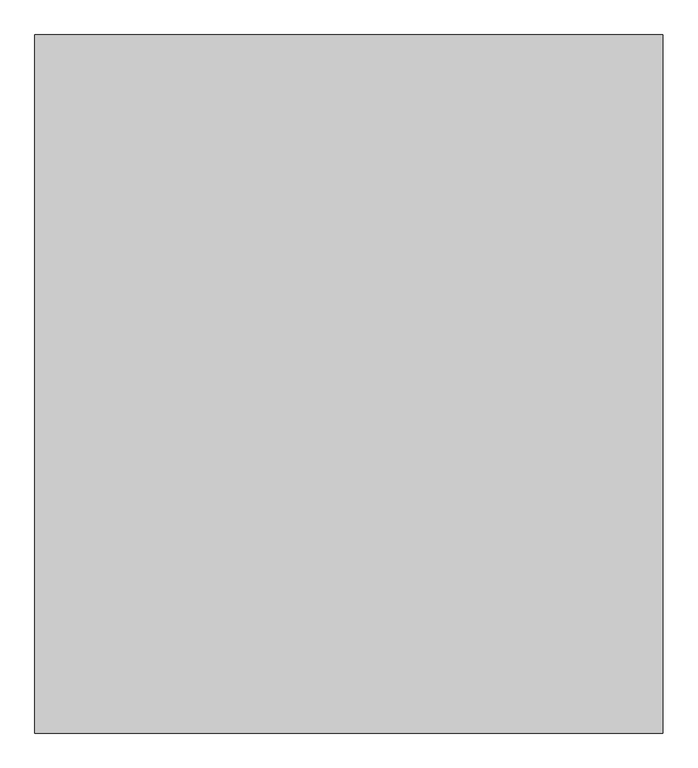
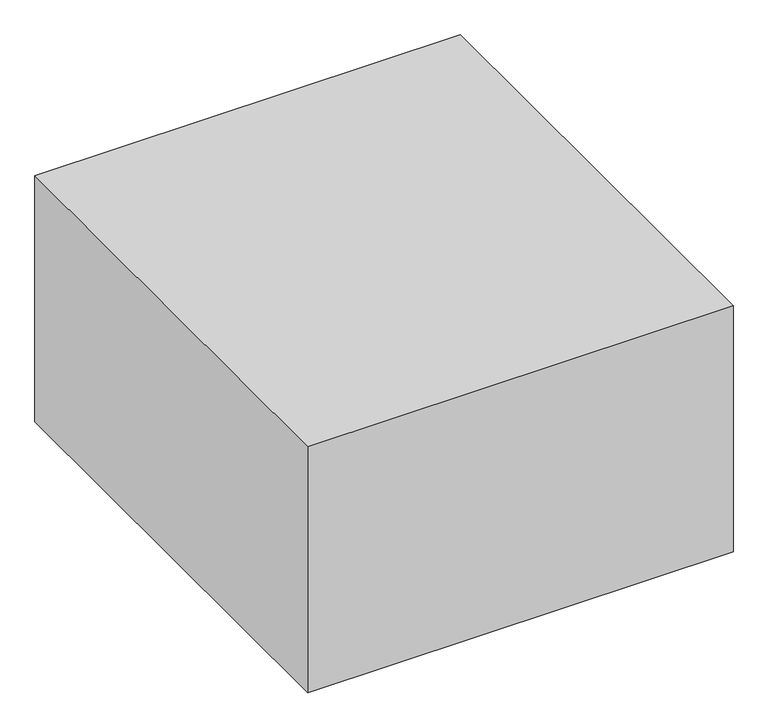
"""IFC4 building model written with IfcOpenShell, lengths in millimetres: proxy geometry, Space Planning Box_hec : Space Planning Box_hec."""

from ifc_helpers import new_model, si_unit, origin, origin_with_axes, place, context, project, spatial, polyline, outline, extrude, source, transform, mapped, element, save


def generic_models_2d265e4a(model_context):
    return source(origin(), model_context, "Body", "SweptSolid", [
        extrude(outline(polyline([(4500.0, 5000.0), (4500.0, -5000.0), (-4500.0, -5000.0), (-4500.0, 5000.0), (4500.0, 5000.0)])), origin_with_axes(), (0.0, 0.0, 1.0), 5500.0),
    ])


if __name__ == "__main__":
    model = new_model("IFC4")
    model_context = context("Model", 3, world=origin())
    ifc_project = project(units=[si_unit("LENGTHUNIT", "METRE", prefix="MILLI")], contexts=[model_context])
    site = spatial("IfcSite", under=ifc_project)
    building = spatial("IfcBuilding", under=site)
    placement = place(None, origin())
    generic_models_shape = generic_models_2d265e4a(model_context)
    element("IfcBuildingElementProxy", 1, Name="Space Planning Box_hec : Space Planning Box_hec", ObjectType="Space Planning Box_hec : Space Planning Box_hec", at=placement, inside=building, context=model_context, shape_type="MappedRepresentation", body=[
        mapped(generic_models_shape, transform((0.0, 0.0, 0.0), x_axis=(1.0, 0.0, 0.0), y_axis=(0.0, 1.0, 0.0), z_axis=(0.0, 0.0, 1.0))),
    ])
    save(model, "model.ifc")

# Revit data of these elements
# Type "Space Planning Box_hec : Space Planning Box_hec"
#   Type Comments = "..."
#   Room Name [instance default] = "?"
#   Interior Finish [instance default] = ""
#   Exterior Finish [instance default] = ""
#   Department [instance default] = ""
#   Assembly Code = "..."
#   ceiling height [instance default] = 0
#   Width [instance default] = 1524 mm
#   Program Area [instance default] = 0.00 m²
#   Length [instance default] = 1524 mm
#   Height [instance default] = 1524 mm
#   Area [instance default] = 2.32258 m²
#   Fill Color [instance default] = Cyan
#   Default Elevation = 0
# Element 1 (IfcBuildingElementProxy, "Space Planning Box_hec : Space Planning Box_hec")
#   Room Name = "Electrical Room (GIS)"
#   Exterior Finish = "N/A..N/A,,EW1..EW2..N/A"
#   Department = "AR"
#   Width = 9000 mm
#   Program Area = 90.00 m²
#   Length = 10000 mm
#   Height = 5500 mm
#   Area = 90.00 m²
#   Materials on its faces: "Cyan"
# Materials
#   "Cyan": class "Generic", colour RGB 0 255 255, transparency 0.2, Cost = 0
